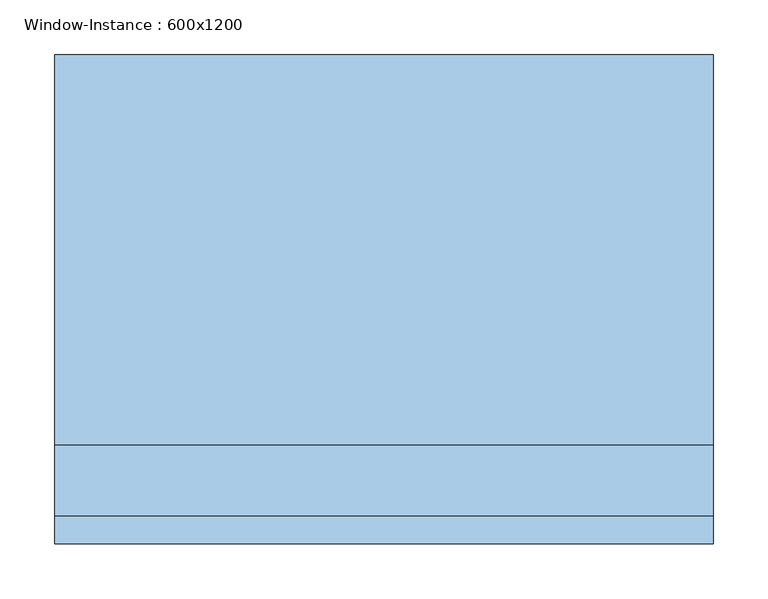
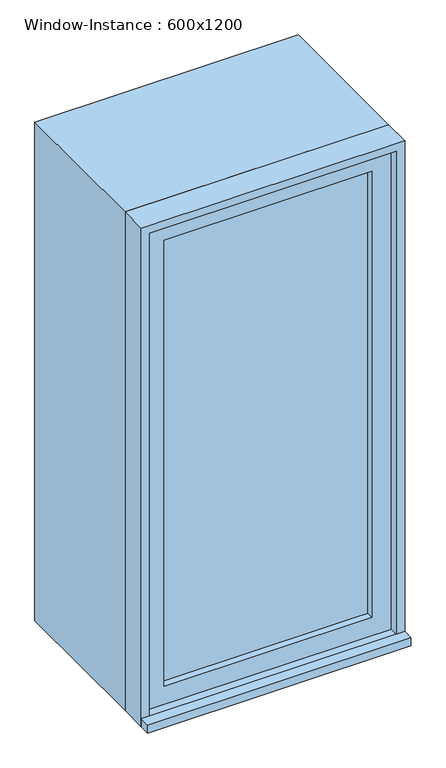
"""IFC4 building model written with IfcOpenShell, lengths in millimetres: window geometry, Window-Instance : 600x1200."""

from ifc_helpers import new_model, si_unit, frame, origin, place, context, project, spatial, polyline, outline, extrude, source, transform, mapped, element, save


def window_instance_600x1200_47b0e0e9(model_context):
    return source(origin(), model_context, "Body", "SweptSolid", [
        extrude(outline(polyline([(-338.1, -235.4), (-338.1, -210.0), (261.9, -210.0), (261.9, -235.4), (-338.1, -235.4)])), frame((0.0, 0.0, 900.0), z_axis=(0.0, 0.0, 1.0), x_axis=(1.0, 0.0, 0.0)), (0.0, 0.0, 1.0), 19.05),
        extrude(outline(polyline([(198.4, -161.425), (198.4, -174.125), (-274.6, -174.125), (-274.6, -161.425), (198.4, -161.425)])), frame((0.0, 0.0, 963.5), z_axis=(0.0, 0.0, 1.0), x_axis=(1.0, 0.0, 0.0)), (0.0, 0.0, 1.0), 1073.0),
        extrude(outline(polyline([(2080.95, -319.05), (919.05, -319.05), (919.05, 242.85), (2080.95, 242.85), (2080.95, -319.05)]), holes=[polyline([(2036.5, -274.6), (2036.5, 198.4), (963.5, 198.4), (963.5, -274.6), (2036.5, -274.6)])]), frame((0.0, -190.0, 0.0), z_axis=(0.0, 1.0, 0.0), x_axis=(0.0, 0.0, 1.0)), (0.0, 0.0, 1.0), 44.45),
        extrude(outline(polyline([(2100.0, -338.1), (900.0, -338.1), (900.0, 261.9), (2100.0, 261.9), (2100.0, -338.1)]), holes=[polyline([(2068.25, -306.35), (2068.25, 230.15), (931.75, 230.15), (931.75, -306.35), (2068.25, -306.35)])]), frame((0.0, -145.55, 0.0), z_axis=(0.0, 1.0, 0.0), x_axis=(0.0, 0.0, 1.0)), (0.0, 0.0, 1.0), 355.55),
        extrude(outline(polyline([(2100.0, 261.9), (2100.0, -338.1), (900.0, -338.1), (900.0, 261.9), (2100.0, 261.9)]), holes=[polyline([(2080.95, 242.85), (919.05, 242.85), (919.05, -319.05), (2080.95, -319.05), (2080.95, 242.85)])]), frame((0.0, -210.0, 0.0), z_axis=(0.0, 1.0, 0.0), x_axis=(0.0, 0.0, 1.0)), (0.0, 0.0, 1.0), 64.45),
    ])


if __name__ == "__main__":
    model = new_model("IFC4")
    model_context = context("Model", 3, world=origin())
    ifc_project = project(units=[si_unit("LENGTHUNIT", "METRE", prefix="MILLI")], contexts=[model_context])
    site = spatial("IfcSite", under=ifc_project)
    building = spatial("IfcBuilding", under=site)
    placement = place(None, origin())
    window_instance_600x1200_shape = window_instance_600x1200_47b0e0e9(model_context)
    element("IfcWindow", 1, ObjectType="Window-Instance : 600x1200", at=placement, inside=building, context=model_context, shape_type="MappedRepresentation", body=[
        mapped(window_instance_600x1200_shape, transform((0.0, 0.0, 0.0), x_axis=(1.0, 0.0, 0.0), y_axis=(0.0, 1.0, 0.0), z_axis=(0.0, 0.0, 1.0))),
    ])
    save(model, "model.ifc")

# Revit data of these elements
# Type "Window-Instance : 600x1200"
#   Type Mark = "7"
#   Construction Type Id = "GSP4R"
#   Assembly Code = "B2020100"
#   Analytic Construction = "1/8 in Pilkington single glazing"
#   Visual Light Transmittance = 0.9
#   Thermal Resistance (R) = 0.149095 (m²·K)/W
#   Solar Heat Gain Coefficient = 0.86
#   Heat Transfer Coefficient (U) = 6.70716 W/(m²·K)
#   Height [instance default] = 1200 mm
#   Default Sill Height = 900 mm
#   Width [instance default] = 600 mm
#   Window Inset = 20 mm
#   Glass Pane Material = WW-EC-GL-Storefront
#   Sash Material = WW-EC-RGB-White
#   Wall Closure = (empty or 0)
# Element 1 (IfcWindow, "Window-Instance : 600x1200")
#   Materials on its faces: "WW-EC-RGB-White", "WW-EC-GL-Storefront"
# Materials
#   "WW-EC-GL-Storefront": class "Glass", colour RGB 236 240 239, transparency 0.85, Description = "Storefront Glass", Cost = 0
#   "WW-EC-RGB-White": class "Generic", colour RGB 255 255 255, transparency 0, Comments = "If region requests off-white, swith asset color to RGB 231-228-220", Description = "Generic Color", Cost = 0
